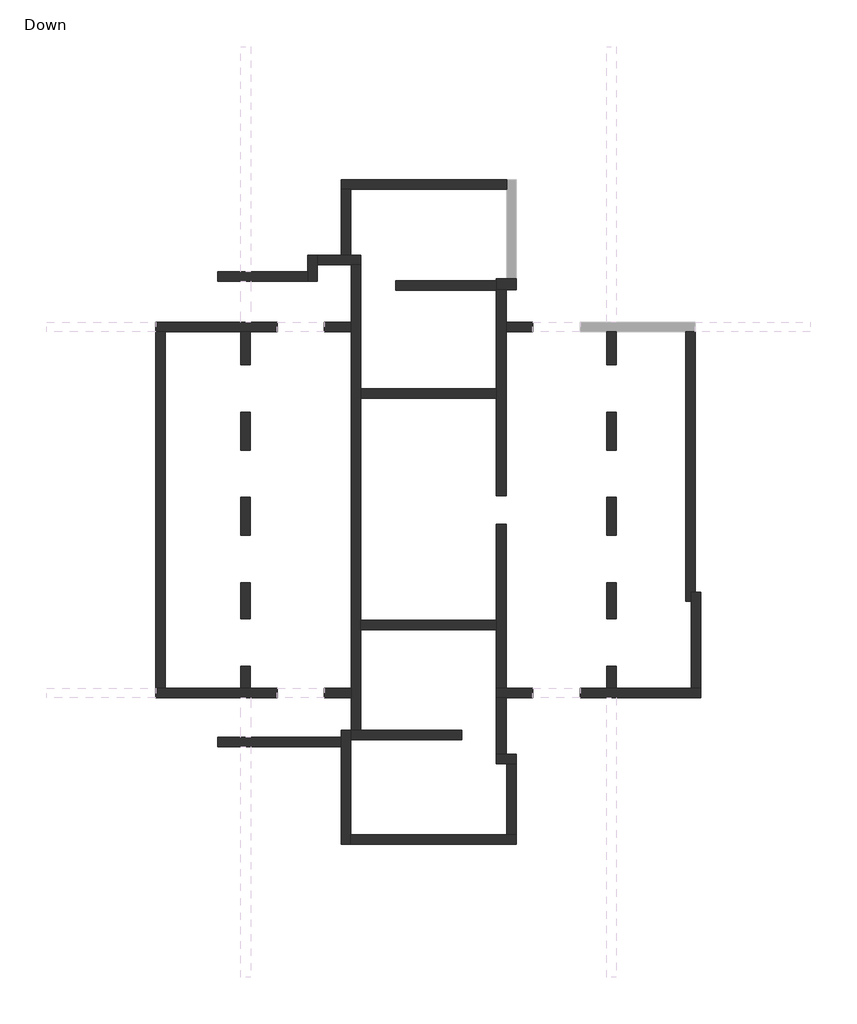
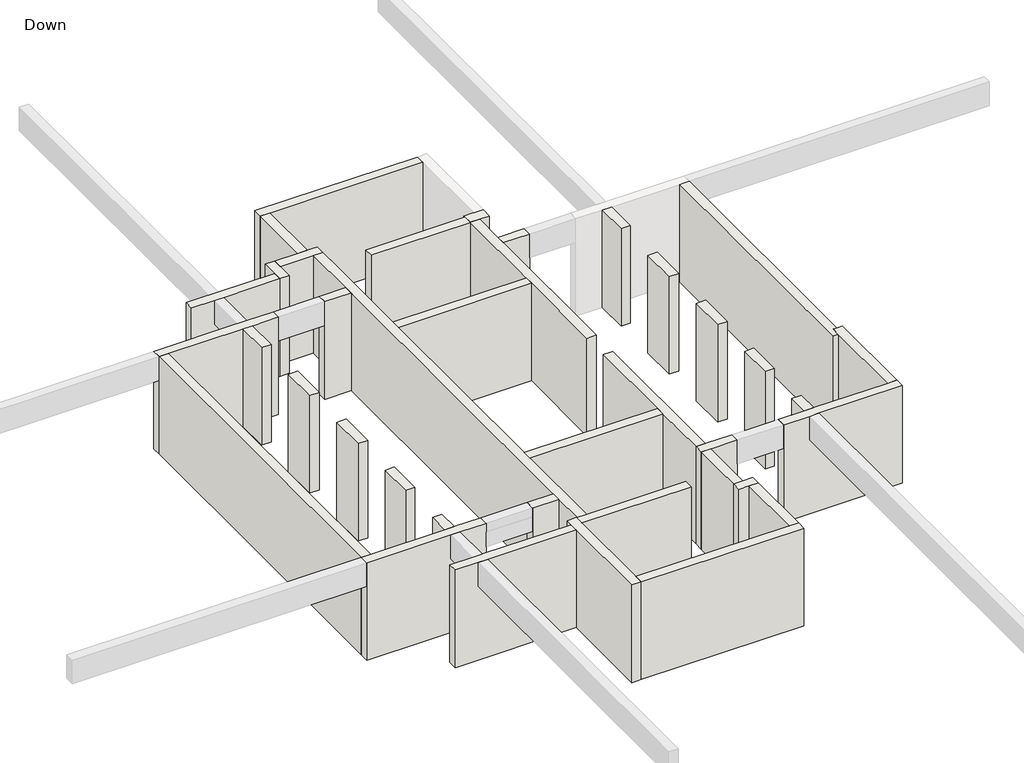
# One storey, part 1 of 2: 39 walls.
"""IFC4 building model written with IfcOpenShell, lengths in millimetres."""

from ifc_helpers import new_model, si_unit, origin, place, context, project, spatial, faceted_brep, element, save

model = new_model("IFC4")

# Units and contexts
model_context = context("Model", 3, world=origin())
ifc_project = project(units=[si_unit("LENGTHUNIT", "METRE", prefix="MILLI")], contexts=[model_context])

# Site, building, storey
site = spatial("IfcSite", under=ifc_project)
building = spatial("IfcBuilding", under=site)
storey = spatial("IfcBuildingStorey", under=building, Name="Down", Elevation=0.0)

# Walls
placement = place(None, origin())
element("IfcWall", 1, ObjectType="30", at=placement, inside=storey, context=model_context, shape_type="Brep", body=[
    faceted_brep([(-9097.9299438, -2256.2642878, 0.0), (-5277.5582989, -2256.2642878, 0.0), (-5277.5582989, -2256.2642878, 2500.0), (-5277.5582989, -2256.2642878, 3000.0), (-5277.5582989, -2256.2642878, 3300.0), (-6115.2243211, -2256.2642878, 3300.0), (-6415.2243211, -2256.2642878, 3300.0), (-9097.9299438, -2256.2642878, 3300.0), (-9097.9299438, -2256.2642878, 2500.0), (-9097.9299438, -1956.2642878, 0.0), (-9097.9299438, -1956.2642878, 2500.0), (-9097.9299438, -1956.2642878, 3300.0), (-8797.9299438, -1956.2642878, 3300.0), (-6419.4715818, -1956.2642878, 3300.0), (-6119.4715818, -1956.2642878, 3300.0), (-5277.5582989, -1956.2642878, 3300.0), (-5277.5582989, -1956.2642878, 2500.0), (-5277.5582989, -1956.2642878, 0.0), (-6119.4715818, -1956.2642878, 0.0), (-6419.4715818, -1956.2642878, 0.0), (-8797.9299438, -1956.2642878, 0.0), (-5277.5582989, -2251.2642878, 3300.0)], [[[0, 1, 2, 3, 4, 5, 6, 7, 8]], [[9, 10, 11, 12, 13, 14, 15, 16, 17, 18, 19, 20]], [[1, 0, 9, 20, 19, 18, 17]], [[4, 3, 2, 1, 17, 16, 15, 21]], [[7, 6, 5, 4, 21, 15, 14, 13, 12, 11]], [[0, 8, 7, 11, 10, 9]]]),
])
element("IfcWall", 2, ObjectType="30", at=placement, inside=storey, context=model_context, shape_type="Brep", body=[
    faceted_brep([(-3791.391747, -2256.2642878, 0.0), (-2947.5514166, -2256.2642878, 0.0), (-2947.5514166, -2256.2642878, 3000.0), (-2947.5514166, -2256.2642878, 3300.0), (-3791.391747, -2256.2642878, 3300.0), (-3791.391747, -2256.2642878, 3000.0), (-3791.391747, -2256.2642878, 2500.0), (-3791.391747, -1956.2642878, 0.0), (-3791.391747, -1956.2642878, 2500.0), (-3791.391747, -1956.2642878, 3300.0), (-2947.5514166, -1956.2642878, 3300.0), (-2947.5514166, -1956.2642878, 3000.0), (-2947.5514166, -1956.2642878, 0.0), (-3791.391747, -2251.2642878, 3300.0)], [[[0, 1, 2, 3, 4, 5, 6]], [[7, 8, 9, 10, 11, 12]], [[1, 0, 7, 12]], [[4, 3, 10, 9, 13]], [[0, 6, 5, 4, 13, 9, 8, 7]], [[3, 2, 1, 12, 11, 10]]]),
])
element("IfcWall", 3, ObjectType="30", at=placement, inside=storey, context=model_context, shape_type="Brep", body=[
    faceted_brep([(-2647.5514166, -3272.2312527, 0.0), (-2647.5514166, -123.5733036, 0.0), (-2647.5514166, 176.4266964, 0.0), (-2647.5514166, 7164.5202959, 0.0), (-2647.5514166, 7464.5202959, 0.0), (-2647.5514166, 11352.4074259, 0.0), (-2647.5514166, 11352.4074259, 3300.0), (-2647.5514166, 10558.9456228, 3300.0), (-2647.5514166, 7464.5202959, 3300.0), (-2647.5514166, 7164.5202959, 3300.0), (-2647.5514166, 176.4266964, 3300.0), (-2647.5514166, -123.5733036, 3300.0), (-2647.5514166, -3272.2312527, 3300.0), (-2947.5514166, -3272.2312527, 0.0), (-2947.5514166, -3272.2312527, 3000.0), (-2947.5514166, -3272.2312527, 3300.0), (-2947.5514166, -2256.2642878, 3300.0), (-2947.5514166, -1956.2642878, 3300.0), (-2947.5514166, 9251.0309634, 3300.0), (-2947.5514166, 9551.0309634, 3300.0), (-2947.5514166, 11352.4074259, 3300.0), (-2947.5514166, 11352.4074259, 3000.0), (-2947.5514166, 11352.4074259, 0.0), (-2947.5514166, 9551.0309634, 0.0), (-2947.5514166, 9251.0309634, 0.0), (-2947.5514166, -1956.2642878, 0.0), (-2947.5514166, -2256.2642878, 0.0)], [[[0, 1, 2, 3, 4, 5, 6, 7, 8, 9, 10, 11, 12]], [[13, 14, 15, 16, 17, 18, 19, 20, 21, 22, 23, 24, 25, 26]], [[5, 4, 3, 2, 1, 0, 13, 26, 25, 24, 23, 22]], [[12, 11, 10, 9, 8, 7, 6, 20, 19, 18, 17, 16, 15]], [[0, 12, 15, 14, 13]], [[6, 5, 22, 21, 20]]]),
])
element("IfcWall", 4, ObjectType="30", at=placement, inside=storey, context=model_context, shape_type="Brep", body=[
    faceted_brep([(-2947.5514166, 9551.0309634, 0.0), (-3791.391747, 9551.0309634, 0.0), (-3791.391747, 9551.0309634, 2500.0), (-3791.391747, 9551.0309634, 3300.0), (-2947.5514166, 9551.0309634, 3300.0), (-2947.5514166, 9551.0309634, 3000.0), (-2947.5514166, 9251.0309634, 0.0), (-2947.5514166, 9251.0309634, 3000.0), (-2947.5514166, 9251.0309634, 3300.0), (-3791.391747, 9251.0309634, 3300.0), (-3791.391747, 9251.0309634, 2500.0), (-3791.391747, 9251.0309634, 0.0)], [[[0, 1, 2, 3, 4, 5]], [[6, 7, 8, 9, 10, 11]], [[1, 0, 6, 11]], [[3, 2, 1, 11, 10, 9]], [[4, 3, 9, 8]], [[0, 5, 4, 8, 7, 6]]]),
])
element("IfcWall", 5, ObjectType="30", at=placement, inside=storey, context=model_context, shape_type="Brep", body=[
    faceted_brep([(-5277.5582989, 9551.0309634, 0.0), (-9097.9299438, 9551.0309634, 0.0), (-9097.9299438, 9551.0309634, 2500.0), (-9097.9299438, 9551.0309634, 3300.0), (-6415.2243211, 9551.0309634, 3300.0), (-6115.2243211, 9551.0309634, 3300.0), (-5277.5582989, 9551.0309634, 3300.0), (-5277.5582989, 9551.0309634, 2500.0), (-5277.5582989, 9251.0309634, 0.0), (-5277.5582989, 9251.0309634, 2500.0), (-5277.5582989, 9251.0309634, 3300.0), (-6119.4715818, 9251.0309634, 3300.0), (-6419.4715818, 9251.0309634, 3300.0), (-8797.9299438, 9251.0309634, 3300.0), (-9097.9299438, 9251.0309634, 3300.0), (-9097.9299438, 9251.0309634, 2500.0), (-9097.9299438, 9251.0309634, 0.0), (-8797.9299438, 9251.0309634, 0.0), (-6419.4715818, 9251.0309634, 0.0), (-6119.4715818, 9251.0309634, 0.0)], [[[0, 1, 2, 3, 4, 5, 6, 7]], [[8, 9, 10, 11, 12, 13, 14, 15, 16, 17, 18, 19]], [[1, 0, 8, 19, 18, 17, 16]], [[6, 5, 4, 3, 14, 13, 12, 11, 10]], [[0, 7, 6, 10, 9, 8]], [[3, 2, 1, 16, 15, 14]]]),
])
element("IfcWall", 6, ObjectType="30", at=placement, inside=storey, context=model_context, shape_type="Brep", body=[
    faceted_brep([(-9097.9299438, 9251.0309634, 0.0), (-9097.9299438, -1956.2642878, 0.0), (-9097.9299438, -1956.2642878, 3000.0), (-9097.9299438, -1956.2642878, 3300.0), (-9097.9299438, 9251.0309634, 3300.0), (-9097.9299438, 9251.0309634, 3000.0), (-8797.9299438, 9251.0309634, 0.0), (-8797.9299438, 9251.0309634, 3300.0), (-8797.9299438, -1956.2642878, 3300.0), (-8797.9299438, -1956.2642878, 0.0)], [[[0, 1, 2, 3, 4, 5]], [[6, 7, 8, 9]], [[1, 0, 6, 9]], [[4, 3, 8, 7]], [[3, 2, 1, 9, 8]], [[0, 5, 4, 7, 6]]]),
])
element("IfcWall", 7, ObjectType="30", at=placement, inside=storey, context=model_context, shape_type="Brep", body=[
    faceted_brep([(-6119.4715818, -1956.2642878, 0.0), (-6119.4715818, -1265.4865865, 0.0), (-6119.4715818, -1265.4865865, 3000.0), (-6119.4715818, -1265.4865865, 3300.0), (-6119.4715818, -1956.2642878, 3300.0), (-6119.4715818, -1956.2642878, 3000.0), (-6419.4715818, -1956.2642878, 0.0), (-6419.4715818, -1956.2642878, 3300.0), (-6419.4715818, -1265.4865865, 3300.0), (-6419.4715818, -1265.4865865, 3000.0), (-6419.4715818, -1265.4865865, 0.0)], [[[0, 1, 2, 3, 4, 5]], [[6, 7, 8, 9, 10]], [[1, 0, 6, 10]], [[3, 2, 1, 10, 9, 8]], [[4, 3, 8, 7]], [[0, 5, 4, 7, 6]]]),
])
element("IfcWall", 8, ObjectType="30", at=placement, inside=storey, context=model_context, shape_type="Brep", body=[
    faceted_brep([(-6119.4715818, 224.8781761, 0.0), (-6119.4715818, 1362.5932484, 0.0), (-6119.4715818, 1362.5932484, 3000.0), (-6119.4715818, 1362.5932484, 3300.0), (-6119.4715818, 224.8781761, 3300.0), (-6119.4715818, 224.8781761, 3000.0), (-6419.4715818, 224.8781761, 0.0), (-6419.4715818, 224.8781761, 3000.0), (-6419.4715818, 224.8781761, 3300.0), (-6419.4715818, 1362.5932484, 3300.0), (-6419.4715818, 1362.5932484, 3000.0), (-6419.4715818, 1362.5932484, 0.0)], [[[0, 1, 2, 3, 4, 5]], [[6, 7, 8, 9, 10, 11]], [[1, 0, 6, 11]], [[3, 2, 1, 11, 10, 9]], [[4, 3, 9, 8]], [[0, 5, 4, 8, 7, 6]]]),
])
element("IfcWall", 9, ObjectType="30", at=placement, inside=storey, context=model_context, shape_type="Brep", body=[
    faceted_brep([(-6119.4715818, 2852.9580109, 0.0), (-6119.4715818, 4041.0516104, 0.0), (-6119.4715818, 4041.0516104, 3000.0), (-6119.4715818, 4041.0516104, 3300.0), (-6119.4715818, 2852.9580109, 3300.0), (-6119.4715818, 2852.9580109, 3000.0), (-6419.4715818, 2852.9580109, 0.0), (-6419.4715818, 2852.9580109, 3000.0), (-6419.4715818, 2852.9580109, 3300.0), (-6419.4715818, 4041.0516104, 3300.0), (-6419.4715818, 4041.0516104, 3000.0), (-6419.4715818, 4041.0516104, 0.0)], [[[0, 1, 2, 3, 4, 5]], [[6, 7, 8, 9, 10, 11]], [[1, 0, 6, 11]], [[3, 2, 1, 11, 10, 9]], [[4, 3, 9, 8]], [[0, 5, 4, 8, 7, 6]]]),
])
element("IfcWall", 10, ObjectType="30", at=placement, inside=storey, context=model_context, shape_type="Brep", body=[
    faceted_brep([(-6119.4715818, 5531.4163729, 0.0), (-6119.4715818, 6719.5099724, 0.0), (-6119.4715818, 6719.5099724, 3000.0), (-6119.4715818, 6719.5099724, 3300.0), (-6119.4715818, 5531.4163729, 3300.0), (-6119.4715818, 5531.4163729, 3000.0), (-6419.4715818, 5531.4163729, 0.0), (-6419.4715818, 5531.4163729, 3000.0), (-6419.4715818, 5531.4163729, 3300.0), (-6419.4715818, 6719.5099724, 3300.0), (-6419.4715818, 6719.5099724, 3000.0), (-6419.4715818, 6719.5099724, 0.0)], [[[0, 1, 2, 3, 4, 5]], [[6, 7, 8, 9, 10, 11]], [[1, 0, 6, 11]], [[3, 2, 1, 11, 10, 9]], [[4, 3, 9, 8]], [[0, 5, 4, 8, 7, 6]]]),
])
element("IfcWall", 11, ObjectType="30", at=placement, inside=storey, context=model_context, shape_type="Brep", body=[
    faceted_brep([(-6119.4715818, 8205.6765243, 0.0), (-6119.4715818, 9251.0309634, 0.0), (-6119.4715818, 9251.0309634, 3000.0), (-6119.4715818, 9251.0309634, 3300.0), (-6119.4715818, 8205.6765243, 3300.0), (-6119.4715818, 8205.6765243, 3000.0), (-6419.4715818, 8205.6765243, 0.0), (-6419.4715818, 8205.6765243, 3000.0), (-6419.4715818, 8205.6765243, 3300.0), (-6419.4715818, 9251.0309634, 3300.0), (-6419.4715818, 9251.0309634, 0.0)], [[[0, 1, 2, 3, 4, 5]], [[6, 7, 8, 9, 10]], [[1, 0, 6, 10]], [[4, 3, 9, 8]], [[0, 5, 4, 8, 7, 6]], [[3, 2, 1, 10, 9]]]),
])
element("IfcWall", 12, ObjectType="30", at=placement, inside=storey, context=model_context, shape_type="Brep", body=[
    faceted_brep([(8042.8271106, -1956.2642878, 0.0), (7742.8271106, -1956.2642878, 0.0), (5384.3687486, -1956.2642878, 0.0), (5084.3687486, -1956.2642878, 0.0), (4242.4554657, -1956.2642878, 0.0), (4242.4554657, -1956.2642878, 2500.0), (4242.4554657, -1956.2642878, 3300.0), (5084.3687486, -1956.2642878, 3300.0), (5384.3687486, -1956.2642878, 3300.0), (7742.8271106, -1956.2642878, 3300.0), (8042.8271106, -1956.2642878, 3300.0), (8042.8271106, -1956.2642878, 2500.0), (8042.8271106, -2256.2642878, 0.0), (8042.8271106, -2256.2642878, 2500.0), (8042.8271106, -2256.2642878, 3300.0), (5373.25294, -2256.2642878, 3300.0), (5073.25294, -2256.2642878, 3300.0), (4242.4554657, -2256.2642878, 3300.0), (4242.4554657, -2256.2642878, 2500.0), (4242.4554657, -2256.2642878, 0.0)], [[[0, 1, 2, 3, 4, 5, 6, 7, 8, 9, 10, 11]], [[12, 13, 14, 15, 16, 17, 18, 19]], [[4, 3, 2, 1, 0, 12, 19]], [[6, 5, 4, 19, 18, 17]], [[10, 9, 8, 7, 6, 17, 16, 15, 14]], [[0, 11, 10, 14, 13, 12]]]),
])
element("IfcWall", 13, ObjectType="30", at=placement, inside=storey, context=model_context, shape_type="Brep", body=[
    faceted_brep([(2756.2889137, -1956.2642878, 0.0), (1915.9035042, -1956.2642878, 0.0), (1615.9035042, -1956.2642878, 0.0), (1615.9035042, -1956.2642878, 3300.0), (1915.9035042, -1956.2642878, 3300.0), (2756.2889137, -1956.2642878, 3300.0), (2756.2889137, -1956.2642878, 2500.0), (2756.2889137, -2256.2642878, 0.0), (2756.2889137, -2256.2642878, 2500.0), (2756.2889137, -2256.2642878, 3300.0), (1915.9035042, -2256.2642878, 3300.0), (1615.9035042, -2256.2642878, 3300.0), (1615.9035042, -2256.2642878, 0.0), (1915.9035042, -2256.2642878, 0.0)], [[[0, 1, 2, 3, 4, 5, 6]], [[7, 8, 9, 10, 11, 12, 13]], [[2, 1, 0, 7, 13, 12]], [[5, 4, 3, 11, 10, 9]], [[0, 6, 5, 9, 8, 7]], [[3, 2, 12, 11]]]),
])
element("IfcWall", 14, ObjectType="30", at=placement, inside=storey, context=model_context, shape_type="Brep", body=[
    faceted_brep([(1915.9035042, -1956.2642878, 0.0), (1915.9035042, 3193.7357122, 0.0), (1915.9035042, 3193.7357122, 3000.0), (1915.9035042, 3193.7357122, 3300.0), (1915.9035042, -1956.2642878, 3300.0), (1915.9035042, -1956.2642878, 3000.0), (1615.9035042, -1956.2642878, 0.0), (1615.9035042, -1956.2642878, 3300.0), (1615.9035042, -123.5733036, 3300.0), (1615.9035042, 176.4266964, 3300.0), (1615.9035042, 3193.7357122, 3300.0), (1615.9035042, 3193.7357122, 3000.0), (1615.9035042, 3193.7357122, 0.0), (1615.9035042, 176.4266964, 0.0), (1615.9035042, -123.5733036, 0.0)], [[[0, 1, 2, 3, 4, 5]], [[6, 7, 8, 9, 10, 11, 12, 13, 14]], [[1, 0, 6, 14, 13, 12]], [[3, 2, 1, 12, 11, 10]], [[4, 3, 10, 9, 8, 7]], [[0, 5, 4, 7, 6]]]),
])
element("IfcWall", 15, ObjectType="30", at=placement, inside=storey, context=model_context, shape_type="Brep", body=[
    faceted_brep([(1915.9035042, 9251.0309634, 0.0), (2756.2889137, 9251.0309634, 0.0), (2756.2889137, 9251.0309634, 2500.0), (2756.2889137, 9251.0309634, 3300.0), (1915.9035042, 9251.0309634, 3300.0), (1915.9035042, 9251.0309634, 3000.0), (1915.9035042, 9551.0309634, 0.0), (1915.9035042, 9551.0309634, 3000.0), (1915.9035042, 9551.0309634, 3300.0), (2756.2889137, 9551.0309634, 3300.0), (2756.2889137, 9551.0309634, 2500.0), (2756.2889137, 9551.0309634, 0.0)], [[[0, 1, 2, 3, 4, 5]], [[6, 7, 8, 9, 10, 11]], [[1, 0, 6, 11]], [[3, 2, 1, 11, 10, 9]], [[4, 3, 9, 8]], [[0, 5, 4, 8, 7, 6]]]),
])
element("IfcWall", 16, ObjectType="30", at=placement, inside=storey, context=model_context, shape_type="Brep", body=[
    faceted_brep([(7742.8271106, 1064.5202959, 0.0), (7742.8271106, 771.0309634, 0.0), (7742.8271106, -1956.2642878, 0.0), (7742.8271106, -1956.2642878, 3300.0), (7742.8271106, 771.0309634, 3300.0), (7742.8271106, 1064.5202959, 3300.0), (8042.8271106, 1064.5202959, 0.0), (8042.8271106, 1064.5202959, 3000.0), (8042.8271106, 1064.5202959, 3300.0), (8042.8271106, -1956.2642878, 3300.0), (8042.8271106, -1956.2642878, 3000.0), (8042.8271106, -1956.2642878, 0.0), (7862.8408752, 1064.5202959, 0.0), (7862.8408752, 1064.5202959, 3300.0)], [[[0, 1, 2, 3, 4, 5]], [[6, 7, 8, 9, 10, 11]], [[2, 1, 0, 12, 6, 11]], [[5, 4, 3, 9, 8, 13]], [[0, 5, 13, 8, 7, 6, 12]], [[3, 2, 11, 10, 9]]]),
])
element("IfcWall", 17, ObjectType="30", at=placement, inside=storey, context=model_context, shape_type="Brep", body=[
    faceted_brep([(5384.3687486, -1956.2642878, 0.0), (5384.3687486, -1265.4865865, 0.0), (5384.3687486, -1265.4865865, 3000.0), (5384.3687486, -1265.4865865, 3300.0), (5384.3687486, -1956.2642878, 3300.0), (5084.3687486, -1956.2642878, 0.0), (5084.3687486, -1956.2642878, 3000.0), (5084.3687486, -1956.2642878, 3300.0), (5084.3687486, -1265.4865865, 3300.0), (5084.3687486, -1265.4865865, 3000.0), (5084.3687486, -1265.4865865, 0.0)], [[[0, 1, 2, 3, 4]], [[5, 6, 7, 8, 9, 10]], [[1, 0, 5, 10]], [[3, 2, 1, 10, 9, 8]], [[4, 3, 8, 7]], [[0, 4, 7, 6, 5]]]),
])
element("IfcWall", 18, ObjectType="30", at=placement, inside=storey, context=model_context, shape_type="Brep", body=[
    faceted_brep([(5384.3687486, 224.8781761, 0.0), (5384.3687486, 1362.5932484, 0.0), (5384.3687486, 1362.5932484, 3000.0), (5384.3687486, 1362.5932484, 3300.0), (5384.3687486, 224.8781761, 3300.0), (5384.3687486, 224.8781761, 3000.0), (5084.3687486, 224.8781761, 0.0), (5084.3687486, 224.8781761, 3000.0), (5084.3687486, 224.8781761, 3300.0), (5084.3687486, 1362.5932484, 3300.0), (5084.3687486, 1362.5932484, 3000.0), (5084.3687486, 1362.5932484, 0.0)], [[[0, 1, 2, 3, 4, 5]], [[6, 7, 8, 9, 10, 11]], [[1, 0, 6, 11]], [[3, 2, 1, 11, 10, 9]], [[4, 3, 9, 8]], [[0, 5, 4, 8, 7, 6]]]),
])
element("IfcWall", 19, ObjectType="30", at=placement, inside=storey, context=model_context, shape_type="Brep", body=[
    faceted_brep([(5384.3687486, 2852.9580109, 0.0), (5384.3687486, 4041.0516104, 0.0), (5384.3687486, 4041.0516104, 3000.0), (5384.3687486, 4041.0516104, 3300.0), (5384.3687486, 2852.9580109, 3300.0), (5384.3687486, 2852.9580109, 3000.0), (5084.3687486, 2852.9580109, 0.0), (5084.3687486, 2852.9580109, 3000.0), (5084.3687486, 2852.9580109, 3300.0), (5084.3687486, 4041.0516104, 3300.0), (5084.3687486, 4041.0516104, 3000.0), (5084.3687486, 4041.0516104, 0.0)], [[[0, 1, 2, 3, 4, 5]], [[6, 7, 8, 9, 10, 11]], [[1, 0, 6, 11]], [[3, 2, 1, 11, 10, 9]], [[4, 3, 9, 8]], [[0, 5, 4, 8, 7, 6]]]),
])
element("IfcWall", 20, ObjectType="30", at=placement, inside=storey, context=model_context, shape_type="Brep", body=[
    faceted_brep([(5384.3687486, 5531.4163729, 0.0), (5384.3687486, 6719.5099724, 0.0), (5384.3687486, 6719.5099724, 3000.0), (5384.3687486, 6719.5099724, 3300.0), (5384.3687486, 5531.4163729, 3300.0), (5384.3687486, 5531.4163729, 3000.0), (5084.3687486, 5531.4163729, 0.0), (5084.3687486, 5531.4163729, 3000.0), (5084.3687486, 5531.4163729, 3300.0), (5084.3687486, 6719.5099724, 3300.0), (5084.3687486, 6719.5099724, 3000.0), (5084.3687486, 6719.5099724, 0.0)], [[[0, 1, 2, 3, 4, 5]], [[6, 7, 8, 9, 10, 11]], [[1, 0, 6, 11]], [[3, 2, 1, 11, 10, 9]], [[4, 3, 9, 8]], [[0, 5, 4, 8, 7, 6]]]),
])
element("IfcWall", 21, ObjectType="30", at=placement, inside=storey, context=model_context, shape_type="Brep", body=[
    faceted_brep([(5384.3687486, 8205.6765243, 0.0), (5384.3687486, 9251.0309634, 0.0), (5384.3687486, 9251.0309634, 3300.0), (5384.3687486, 8205.6765243, 3300.0), (5384.3687486, 8205.6765243, 3000.0), (5084.3687486, 8205.6765243, 0.0), (5084.3687486, 8205.6765243, 3000.0), (5084.3687486, 8205.6765243, 3300.0), (5084.3687486, 9251.0309634, 3300.0), (5084.3687486, 9251.0309634, 3000.0), (5084.3687486, 9251.0309634, 0.0)], [[[0, 1, 2, 3, 4]], [[5, 6, 7, 8, 9, 10]], [[1, 0, 5, 10]], [[3, 2, 8, 7]], [[0, 4, 3, 7, 6, 5]], [[2, 1, 10, 9, 8]]]),
])
element("IfcWall", 22, ObjectType="30", at=placement, inside=storey, context=model_context, shape_type="Brep", body=[
    faceted_brep([(7562.8408752, 9251.0309634, 0.0), (7562.8408752, 771.0309634, 0.0), (7562.8408752, 771.0309634, 3300.0), (7562.8408752, 9251.0309634, 3300.0), (7862.8408752, 9251.0309634, 0.0), (7862.8408752, 9251.0309634, 3000.0), (7862.8408752, 9251.0309634, 3300.0), (7862.8408752, 1064.5202959, 3300.0), (7862.8408752, 1064.5202959, 3000.0), (7862.8408752, 1064.5202959, 0.0), (7742.8271106, 1064.5202959, 0.0), (7742.8271106, 771.0309634, 0.0), (7742.8271106, 771.0309634, 3300.0), (7742.8271106, 1064.5202959, 3300.0)], [[[0, 1, 2, 3]], [[4, 5, 6, 7, 8, 9]], [[1, 0, 4, 9, 10, 11]], [[2, 1, 11, 12]], [[3, 2, 12, 13, 7, 6]], [[0, 3, 6, 5, 4]], [[10, 13, 12, 11]], [[13, 10, 9, 8, 7]]]),
])
element("IfcWall", 23, ObjectType="30", at=placement, inside=storey, context=model_context, shape_type="Brep", body=[
    faceted_brep([(-2647.5514166, -123.5733036, 0.0), (1615.9035042, -123.5733036, 0.0), (1615.9035042, -123.5733036, 3300.0), (-2647.5514166, -123.5733036, 3300.0), (-2647.5514166, 176.4266964, 0.0), (-2647.5514166, 176.4266964, 3000.0), (-2647.5514166, 176.4266964, 3300.0), (1615.9035042, 176.4266964, 3300.0), (1615.9035042, 176.4266964, 3000.0), (1615.9035042, 176.4266964, 0.0)], [[[0, 1, 2, 3]], [[4, 5, 6, 7, 8, 9]], [[1, 0, 4, 9]], [[3, 2, 7, 6]], [[0, 3, 6, 5, 4]], [[2, 1, 9, 8, 7]]]),
])
element("IfcWall", 24, ObjectType="30", at=placement, inside=storey, context=model_context, shape_type="Brep", body=[
    faceted_brep([(-7145.7620154, -3792.8093669, 0.0), (-3270.8136327, -3792.8093669, 0.0), (-3270.8136327, -3792.8093669, 3000.0), (-3270.8136327, -3792.8093669, 3300.0), (-6115.2243211, -3792.8093669, 3300.0), (-6415.2243211, -3792.8093669, 3300.0), (-7145.7620154, -3792.8093669, 3300.0), (-7145.7620154, -3792.8093669, 3000.0), (-7145.7620154, -3492.8093669, 0.0), (-7145.7620154, -3492.8093669, 3000.0), (-7145.7620154, -3492.8093669, 3300.0), (-6415.2243211, -3492.8093669, 3300.0), (-6115.2243211, -3492.8093669, 3300.0), (-3270.8136327, -3492.8093669, 3300.0), (-3270.8136327, -3492.8093669, 3000.0), (-3270.8136327, -3492.8093669, 0.0)], [[[0, 1, 2, 3, 4, 5, 6, 7]], [[8, 9, 10, 11, 12, 13, 14, 15]], [[1, 0, 8, 15]], [[6, 5, 4, 3, 13, 12, 11, 10]], [[0, 7, 6, 10, 9, 8]], [[3, 2, 1, 15, 14, 13]]]),
])
element("IfcWall", 25, ObjectType="30", at=placement, inside=storey, context=model_context, shape_type="Brep", body=[
    faceted_brep([(-3270.8136327, -3272.2312527, 0.0), (-3270.8136327, -3492.8093669, 0.0), (-3270.8136327, -3792.8093669, 0.0), (-3270.8136327, -6865.8995252, 0.0), (-3270.8136327, -6865.8995252, 3000.0), (-3270.8136327, -6865.8995252, 3300.0), (-3270.8136327, -3792.8093669, 3300.0), (-3270.8136327, -3492.8093669, 3300.0), (-3270.8136327, -3272.2312527, 3300.0), (-3270.8136327, -3272.2312527, 3000.0), (-2970.8136327, -3272.2312527, 0.0), (-2970.8136327, -3272.2312527, 3300.0), (-2970.8136327, -3572.2312527, 3300.0), (-2970.8136327, -6565.8995252, 3300.0), (-2970.8136327, -6865.8995252, 3300.0), (-2970.8136327, -6865.8995252, 0.0), (-2970.8136327, -6565.8995252, 0.0), (-2970.8136327, -3572.2312527, 0.0)], [[[0, 1, 2, 3, 4, 5, 6, 7, 8, 9]], [[10, 11, 12, 13, 14, 15, 16, 17]], [[3, 2, 1, 0, 10, 17, 16, 15]], [[8, 7, 6, 5, 14, 13, 12, 11]], [[5, 4, 3, 15, 14]], [[0, 9, 8, 11, 10]]]),
])
element("IfcWall", 26, ObjectType="30", at=placement, inside=storey, context=model_context, shape_type="Brep", body=[
    faceted_brep([(-2970.8136327, -6865.8995252, 0.0), (2233.0404623, -6865.8995252, 0.0), (2233.0404623, -6865.8995252, 3000.0), (2233.0404623, -6865.8995252, 3300.0), (-2970.8136327, -6865.8995252, 3300.0), (-2970.8136327, -6565.8995252, 0.0), (-2970.8136327, -6565.8995252, 3000.0), (-2970.8136327, -6565.8995252, 3300.0), (1933.0404623, -6565.8995252, 3300.0), (2233.0404623, -6565.8995252, 3300.0), (2233.0404623, -6565.8995252, 0.0), (1933.0404623, -6565.8995252, 0.0)], [[[0, 1, 2, 3, 4]], [[5, 6, 7, 8, 9, 10, 11]], [[1, 0, 5, 11, 10]], [[4, 3, 9, 8, 7]], [[0, 4, 7, 6, 5]], [[3, 2, 1, 10, 9]]]),
])
element("IfcWall", 27, ObjectType="30", at=placement, inside=storey, context=model_context, shape_type="Brep", body=[
    faceted_brep([(2233.0404623, -6565.8995252, 0.0), (2233.0404623, -4336.2642878, 0.0), (2233.0404623, -4336.2642878, 3300.0), (2233.0404623, -6565.8995252, 3300.0), (1933.0404623, -6565.8995252, 0.0), (1933.0404623, -6565.8995252, 3000.0), (1933.0404623, -6565.8995252, 3300.0), (1933.0404623, -4336.2642878, 3300.0), (1933.0404623, -4336.2642878, 3000.0), (1933.0404623, -4336.2642878, 0.0)], [[[0, 1, 2, 3]], [[4, 5, 6, 7, 8, 9]], [[1, 0, 4, 9]], [[3, 2, 7, 6]], [[0, 3, 6, 5, 4]], [[2, 1, 9, 8, 7]]]),
])
element("IfcWall", 28, ObjectType="30", at=placement, inside=storey, context=model_context, shape_type="Brep", body=[
    faceted_brep([(1615.9035042, -2256.2642878, 0.0), (1615.9035042, -4036.2642878, 0.0), (1615.9035042, -4036.2642878, 3300.0), (1615.9035042, -3272.2312527, 3300.0), (1615.9035042, -2256.2642878, 3300.0), (1915.9035042, -2256.2642878, 0.0), (1915.9035042, -2256.2642878, 3000.0), (1915.9035042, -2256.2642878, 3300.0), (1915.9035042, -4036.2642878, 3300.0), (1915.9035042, -4036.2642878, 3000.0), (1915.9035042, -4036.2642878, 0.0)], [[[0, 1, 2, 3, 4]], [[5, 6, 7, 8, 9, 10]], [[1, 0, 5, 10]], [[4, 3, 2, 8, 7]], [[0, 4, 7, 6, 5]], [[2, 1, 10, 9, 8]]]),
])
element("IfcWall", 29, ObjectType="30", at=placement, inside=storey, context=model_context, shape_type="Brep", body=[
    faceted_brep([(1615.9035042, -4336.2642878, 0.0), (1933.0404623, -4336.2642878, 0.0), (2233.0404623, -4336.2642878, 0.0), (2233.0404623, -4336.2642878, 3300.0), (1933.0404623, -4336.2642878, 3300.0), (1615.9035042, -4336.2642878, 3300.0), (1615.9035042, -4336.2642878, 3000.0), (1615.9035042, -4036.2642878, 0.0), (1615.9035042, -4036.2642878, 3300.0), (1915.9035042, -4036.2642878, 3300.0), (2233.0404623, -4036.2642878, 3300.0), (2233.0404623, -4036.2642878, 3000.0), (2233.0404623, -4036.2642878, 0.0), (1915.9035042, -4036.2642878, 0.0)], [[[0, 1, 2, 3, 4, 5, 6]], [[7, 8, 9, 10, 11, 12, 13]], [[2, 1, 0, 7, 13, 12]], [[5, 4, 3, 10, 9, 8]], [[0, 6, 5, 8, 7]], [[3, 2, 12, 11, 10]]]),
])
element("IfcWall", 30, ObjectType="30", at=placement, inside=storey, context=model_context, shape_type="Brep", body=[
    faceted_brep([(1915.9035042, 4091.4301376, 0.0), (1915.9035042, 9251.0309634, 0.0), (1915.9035042, 9551.0309634, 0.0), (1915.9035042, 10565.0708809, 0.0), (1915.9035042, 10565.0708809, 3000.0), (1915.9035042, 10565.0708809, 3300.0), (1915.9035042, 9551.0309634, 3300.0), (1915.9035042, 9251.0309634, 3300.0), (1915.9035042, 4091.4301376, 3300.0), (1915.9035042, 4091.4301376, 3000.0), (1615.9035042, 4091.4301376, 0.0), (1615.9035042, 4091.4301376, 3000.0), (1615.9035042, 4091.4301376, 3300.0), (1615.9035042, 7164.5202959, 3300.0), (1615.9035042, 7464.5202959, 3300.0), (1615.9035042, 10558.9456228, 3300.0), (1615.9035042, 10565.0708809, 3300.0), (1615.9035042, 10565.0708809, 0.0), (1615.9035042, 10558.9456228, 0.0), (1615.9035042, 7464.5202959, 0.0), (1615.9035042, 7164.5202959, 0.0)], [[[0, 1, 2, 3, 4, 5, 6, 7, 8, 9]], [[10, 11, 12, 13, 14, 15, 16, 17, 18, 19, 20]], [[3, 2, 1, 0, 10, 20, 19, 18, 17]], [[8, 7, 6, 5, 16, 15, 14, 13, 12]], [[0, 9, 8, 12, 11, 10]], [[5, 4, 3, 17, 16]]]),
])
element("IfcWall", 31, ObjectType="30", at=placement, inside=storey, context=model_context, shape_type="Brep", body=[
    faceted_brep([(-2647.5514166, 7164.5202959, 0.0), (1615.9035042, 7164.5202959, 0.0), (1615.9035042, 7164.5202959, 3000.0), (1615.9035042, 7164.5202959, 3300.0), (-2647.5514166, 7164.5202959, 3300.0), (-2647.5514166, 7164.5202959, 3000.0), (-2647.5514166, 7464.5202959, 0.0), (-2647.5514166, 7464.5202959, 3300.0), (1615.9035042, 7464.5202959, 3300.0), (1615.9035042, 7464.5202959, 0.0)], [[[0, 1, 2, 3, 4, 5]], [[6, 7, 8, 9]], [[1, 0, 6, 9]], [[4, 3, 8, 7]], [[0, 5, 4, 7, 6]], [[3, 2, 1, 9, 8]]]),
])
element("IfcWall", 32, ObjectType="30", at=placement, inside=storey, context=model_context, shape_type="Brep", body=[
    faceted_brep([(1933.0404623, 14032.7928354, 0.0), (-3270.8136327, 14032.7928354, 0.0), (-3270.8136327, 14032.7928354, 3000.0), (-3270.8136327, 14032.7928354, 3300.0), (1933.0404623, 14032.7928354, 3300.0), (1933.0404623, 13732.7928354, 0.0), (1933.0404623, 13732.7928354, 3000.0), (1933.0404623, 13732.7928354, 3300.0), (-2970.8136327, 13732.7928354, 3300.0), (-3270.8136327, 13732.7928354, 3300.0), (-3270.8136327, 13732.7928354, 0.0), (-2970.8136327, 13732.7928354, 0.0)], [[[0, 1, 2, 3, 4]], [[5, 6, 7, 8, 9, 10, 11]], [[1, 0, 5, 11, 10]], [[4, 3, 9, 8, 7]], [[0, 4, 7, 6, 5]], [[3, 2, 1, 10, 9]]]),
])
element("IfcWall", 33, ObjectType="30", at=placement, inside=storey, context=model_context, shape_type="Brep", body=[
    faceted_brep([(-3270.8136327, 13732.7928354, 0.0), (-3270.8136327, 11652.4074259, 0.0), (-3270.8136327, 11652.4074259, 3000.0), (-3270.8136327, 11652.4074259, 3300.0), (-3270.8136327, 13732.7928354, 3300.0), (-2970.8136327, 13732.7928354, 0.0), (-2970.8136327, 13732.7928354, 3000.0), (-2970.8136327, 13732.7928354, 3300.0), (-2970.8136327, 11652.4074259, 3300.0), (-2970.8136327, 11652.4074259, 3000.0), (-2970.8136327, 11652.4074259, 0.0)], [[[0, 1, 2, 3, 4]], [[5, 6, 7, 8, 9, 10]], [[1, 0, 5, 10]], [[4, 3, 8, 7]], [[0, 4, 7, 6, 5]], [[3, 2, 1, 10, 9, 8]]]),
])
element("IfcWall", 34, ObjectType="30", at=placement, inside=storey, context=model_context, shape_type="Brep", body=[
    faceted_brep([(-2647.5514166, 11652.4074259, 0.0), (-2970.8136327, 11652.4074259, 0.0), (-3270.8136327, 11652.4074259, 0.0), (-4013.8969087, 11652.4074259, 0.0), (-4013.8969087, 11652.4074259, 3300.0), (-3270.8136327, 11652.4074259, 3300.0), (-2970.8136327, 11652.4074259, 3300.0), (-2647.5514166, 11652.4074259, 3300.0), (-2647.5514166, 11652.4074259, 3000.0), (-2647.5514166, 11352.4074259, 0.0), (-2647.5514166, 11352.4074259, 3300.0), (-2947.5514166, 11352.4074259, 3300.0), (-4013.8969087, 11352.4074259, 3300.0), (-4013.8969087, 11352.4074259, 3000.0), (-4013.8969087, 11352.4074259, 0.0), (-2947.5514166, 11352.4074259, 0.0)], [[[0, 1, 2, 3, 4, 5, 6, 7, 8]], [[9, 10, 11, 12, 13, 14, 15]], [[3, 2, 1, 0, 9, 15, 14]], [[7, 6, 5, 4, 12, 11, 10]], [[4, 3, 14, 13, 12]], [[0, 8, 7, 10, 9]]]),
])
element("IfcWall", 35, ObjectType="30", at=placement, inside=storey, context=model_context, shape_type="Brep", body=[
    faceted_brep([(-4013.8969087, 10837.9545698, 0.0), (-4013.8969087, 11352.4074259, 0.0), (-4013.8969087, 11652.4074259, 0.0), (-4013.8969087, 11652.4074259, 3300.0), (-4013.8969087, 11352.4074259, 3300.0), (-4013.8969087, 10837.9545698, 3300.0), (-4013.8969087, 10837.9545698, 3000.0), (-4313.8969087, 10837.9545698, 0.0), (-4313.8969087, 10837.9545698, 3300.0), (-4313.8969087, 11137.9545698, 3300.0), (-4313.8969087, 11652.4074259, 3300.0), (-4313.8969087, 11652.4074259, 3000.0), (-4313.8969087, 11652.4074259, 0.0), (-4313.8969087, 11137.9545698, 0.0)], [[[0, 1, 2, 3, 4, 5, 6]], [[7, 8, 9, 10, 11, 12, 13]], [[2, 1, 0, 7, 13, 12]], [[5, 4, 3, 10, 9, 8]], [[3, 2, 12, 11, 10]], [[0, 6, 5, 8, 7]]]),
])
element("IfcWall", 36, ObjectType="30", at=placement, inside=storey, context=model_context, shape_type="Brep", body=[
    faceted_brep([(-4313.8969087, 11137.9545698, 0.0), (-7145.7620154, 11137.9545698, 0.0), (-7145.7620154, 11137.9545698, 3000.0), (-7145.7620154, 11137.9545698, 3300.0), (-6415.2243211, 11137.9545698, 3300.0), (-6115.2243211, 11137.9545698, 3300.0), (-4313.8969087, 11137.9545698, 3300.0), (-4313.8969087, 11137.9545698, 3000.0), (-4313.8969087, 10837.9545698, 0.0), (-4313.8969087, 10837.9545698, 3300.0), (-6115.2243211, 10837.9545698, 3300.0), (-6415.2243211, 10837.9545698, 3300.0), (-7145.7620154, 10837.9545698, 3300.0), (-7145.7620154, 10837.9545698, 3000.0), (-7145.7620154, 10837.9545698, 0.0)], [[[0, 1, 2, 3, 4, 5, 6, 7]], [[8, 9, 10, 11, 12, 13, 14]], [[1, 0, 8, 14]], [[3, 2, 1, 14, 13, 12]], [[6, 5, 4, 3, 12, 11, 10, 9]], [[0, 7, 6, 9, 8]]]),
])
element("IfcWall", 37, ObjectType="30", at=placement, inside=storey, context=model_context, shape_type="Brep", body=[
    faceted_brep([(-2970.8136327, -3572.2312527, 0.0), (524.3687486, -3572.2312527, 0.0), (524.3687486, -3572.2312527, 3000.0), (524.3687486, -3572.2312527, 3300.0), (-2970.8136327, -3572.2312527, 3300.0), (-2970.8136327, -3572.2312527, 3000.0), (-2970.8136327, -3272.2312527, 0.0), (-2970.8136327, -3272.2312527, 3300.0), (-2947.5514166, -3272.2312527, 3300.0), (-2647.5514166, -3272.2312527, 3300.0), (524.3687486, -3272.2312527, 3300.0), (524.3687486, -3272.2312527, 3000.0), (524.3687486, -3272.2312527, 0.0), (-2647.5514166, -3272.2312527, 0.0), (-2947.5514166, -3272.2312527, 0.0)], [[[0, 1, 2, 3, 4, 5]], [[6, 7, 8, 9, 10, 11, 12, 13, 14]], [[1, 0, 6, 14, 13, 12]], [[3, 2, 1, 12, 11, 10]], [[4, 3, 10, 9, 8, 7]], [[0, 5, 4, 7, 6]]]),
])
element("IfcWall", 38, ObjectType="30", at=placement, inside=storey, context=model_context, shape_type="Brep", body=[
    faceted_brep([(1615.9035042, 10858.9456228, 0.0), (-1557.9437084, 10858.9456228, 0.0), (-1557.9437084, 10858.9456228, 3000.0), (-1557.9437084, 10858.9456228, 3300.0), (1615.9035042, 10858.9456228, 3300.0), (1615.9035042, 10858.9456228, 3000.0), (1615.9035042, 10558.9456228, 0.0), (1615.9035042, 10558.9456228, 3300.0), (-1557.9437084, 10558.9456228, 3300.0), (-1557.9437084, 10558.9456228, 3000.0), (-1557.9437084, 10558.9456228, 0.0), (1615.9035042, 10565.0708809, 0.0), (1615.9035042, 10565.0708809, 3300.0)], [[[0, 1, 2, 3, 4, 5]], [[6, 7, 8, 9, 10]], [[1, 0, 11, 6, 10]], [[3, 2, 1, 10, 9, 8]], [[4, 3, 8, 7, 12]], [[0, 5, 4, 12, 7, 6, 11]]]),
])
element("IfcWall", 39, ObjectType="35", at=placement, inside=storey, context=model_context, shape_type="Brep", body=[
    faceted_brep([(2233.0404623, 10915.0708809, 0.0), (1933.0404623, 10915.0708809, 0.0), (1615.9035042, 10915.0708809, 0.0), (1615.9035042, 10915.0708809, 3000.0), (1615.9035042, 10915.0708809, 3300.0), (1933.0404623, 10915.0708809, 3300.0), (2233.0404623, 10915.0708809, 3300.0), (2233.0404623, 10565.0708809, 0.0), (2233.0404623, 10565.0708809, 3000.0), (2233.0404623, 10565.0708809, 3300.0), (1915.9035042, 10565.0708809, 3300.0), (1615.9035042, 10565.0708809, 3300.0), (1615.9035042, 10565.0708809, 0.0), (1915.9035042, 10565.0708809, 0.0), (1615.9035042, 10858.9456228, 0.0), (1615.9035042, 10858.9456228, 3300.0)], [[[0, 1, 2, 3, 4, 5, 6]], [[7, 8, 9, 10, 11, 12, 13]], [[2, 1, 0, 7, 13, 12, 14]], [[6, 5, 4, 15, 11, 10, 9]], [[4, 3, 2, 14, 12, 11, 15]], [[0, 6, 9, 8, 7]]]),
])

save(model, "model.ifc")

# Revit data of these elements
# Project information
#   Project Issue Date = "Issue Date"
#   Project Status = "Project Status"
#   Client Name = "לקוח"
#   Project Address = "Enter address here"
#   Project Name = "Project 004"
#   Project Number = "מספר פרויקט"
# Type "30"
#   Layers, outside or top first: 30 cm "Concrete" (function 1)
# Type "35"
#   Layers, outside or top first: 35 cm "Concrete" (function 1)
# Element 1 (IfcWall, "30")
#   Comments = ""
#   Mark = "W1"
#   SOFiSTiK_EdgeZones = "W1"
#   SOFiSTiK_AMG_Comments = ""
#   Top Offset = 0 cm
#   Base Offset = 0 cm
#   wall height = 330 cm
#   SOFiSTiK_AMG_Scheduled = yes
#   SOFiSTiK_AMG_Adjusted = yes
#   Phase Created = New Construction
#   Base Constraint = Down
#   Top Constraint = Typical Floor
#   Materials on its faces: "Concrete"
# Element 2 (IfcWall, "30")
#   Comments = ""
#   Mark = "W2"
#   SOFiSTiK_EdgeZones = "W2"
#   SOFiSTiK_AMG_Comments = ""
#   Top Offset = 0 cm
#   Base Offset = 0 cm
#   wall height = 330 cm
#   SOFiSTiK_AMG_Scheduled = yes
#   SOFiSTiK_AMG_Adjusted = yes
#   Phase Created = New Construction
#   Base Constraint = Down
#   Top Constraint = Typical Floor
#   Materials on its faces: "Concrete"
# Element 3 (IfcWall, "30")
#   Comments = ""
#   Mark = "W3"
#   SOFiSTiK_EdgeZones = "W3"
#   SOFiSTiK_AMG_Comments = ""
#   Top Offset = 0 cm
#   Base Offset = 0 cm
#   wall height = 330 cm
#   SOFiSTiK_AMG_Scheduled = yes
#   SOFiSTiK_AMG_Adjusted = yes
#   Phase Created = New Construction
#   Base Constraint = Down
#   Top Constraint = Typical Floor
#   Materials on its faces: "Concrete"
# Element 4 (IfcWall, "30")
#   Comments = ""
#   Mark = "W4"
#   SOFiSTiK_EdgeZones = "W4"
#   SOFiSTiK_AMG_Comments = ""
#   Top Offset = 0 cm
#   Base Offset = 0 cm
#   wall height = 330 cm
#   SOFiSTiK_AMG_Scheduled = yes
#   SOFiSTiK_AMG_Adjusted = yes
#   Phase Created = New Construction
#   Base Constraint = Down
#   Top Constraint = Typical Floor
#   Materials on its faces: "Concrete"
# Element 5 (IfcWall, "30")
#   Comments = ""
#   Mark = "W5"
#   SOFiSTiK_EdgeZones = "W5"
#   SOFiSTiK_AMG_Comments = ""
#   Top Offset = 0 cm
#   Base Offset = 0 cm
#   wall height = 330 cm
#   SOFiSTiK_AMG_Scheduled = yes
#   SOFiSTiK_AMG_Adjusted = yes
#   Phase Created = New Construction
#   Base Constraint = Down
#   Top Constraint = Typical Floor
#   Materials on its faces: "Concrete"
# Element 6 (IfcWall, "30")
#   Comments = ""
#   Mark = "W6"
#   SOFiSTiK_EdgeZones = "W6"
#   SOFiSTiK_AMG_Comments = ""
#   Top Offset = 0 cm
#   Base Offset = 0 cm
#   wall height = 330 cm
#   SOFiSTiK_AMG_Scheduled = yes
#   SOFiSTiK_AMG_Adjusted = yes
#   Phase Created = New Construction
#   Base Constraint = Down
#   Top Constraint = Typical Floor
#   Materials on its faces: "Concrete"
# Element 7 (IfcWall, "30")
#   Comments = ""
#   Mark = "W7"
#   SOFiSTiK_EdgeZones = "W7"
#   SOFiSTiK_AMG_Comments = ""
#   Top Offset = 0 cm
#   Base Offset = 0 cm
#   wall height = 330 cm
#   SOFiSTiK_AMG_Scheduled = yes
#   SOFiSTiK_AMG_Adjusted = yes
#   Phase Created = New Construction
#   Base Constraint = Down
#   Top Constraint = Typical Floor
#   Materials on its faces: "Concrete"
# Element 8 (IfcWall, "30")
#   Comments = ""
#   Mark = "W8"
#   SOFiSTiK_EdgeZones = "W8"
#   SOFiSTiK_AMG_Comments = ""
#   Top Offset = 0 cm
#   Base Offset = 0 cm
#   wall height = 330 cm
#   SOFiSTiK_AMG_Scheduled = yes
#   SOFiSTiK_AMG_Adjusted = yes
#   Phase Created = New Construction
#   Base Constraint = Down
#   Top Constraint = Typical Floor
#   Materials on its faces: "Concrete"
# Element 9 (IfcWall, "30")
#   Comments = ""
#   Mark = "W9"
#   SOFiSTiK_EdgeZones = "W9"
#   SOFiSTiK_AMG_Comments = ""
#   Top Offset = 0 cm
#   Base Offset = 0 cm
#   wall height = 330 cm
#   SOFiSTiK_AMG_Scheduled = yes
#   SOFiSTiK_AMG_Adjusted = yes
#   Phase Created = New Construction
#   Base Constraint = Down
#   Top Constraint = Typical Floor
#   Materials on its faces: "Concrete"
# Element 10 (IfcWall, "30")
#   Comments = ""
#   Mark = "W10"
#   SOFiSTiK_EdgeZones = "W10"
#   SOFiSTiK_AMG_Comments = ""
#   Top Offset = 0 cm
#   Base Offset = 0 cm
#   wall height = 330 cm
#   SOFiSTiK_AMG_Scheduled = yes
#   SOFiSTiK_AMG_Adjusted = yes
#   Phase Created = New Construction
#   Base Constraint = Down
#   Top Constraint = Typical Floor
#   Materials on its faces: "Concrete"
# Element 11 (IfcWall, "30")
#   Comments = ""
#   Mark = "W11"
#   SOFiSTiK_EdgeZones = "W11"
#   SOFiSTiK_AMG_Comments = ""
#   Top Offset = 0 cm
#   Base Offset = 0 cm
#   wall height = 330 cm
#   SOFiSTiK_AMG_Scheduled = yes
#   SOFiSTiK_AMG_Adjusted = yes
#   Phase Created = New Construction
#   Base Constraint = Down
#   Top Constraint = Typical Floor
#   Materials on its faces: "Concrete"
# Element 12 (IfcWall, "30")
#   Comments = ""
#   Mark = "W12"
#   SOFiSTiK_EdgeZones = "W12"
#   SOFiSTiK_AMG_Comments = ""
#   Top Offset = 0 cm
#   Base Offset = 0 cm
#   wall height = 330 cm
#   SOFiSTiK_AMG_Scheduled = yes
#   SOFiSTiK_AMG_Adjusted = yes
#   Phase Created = New Construction
#   Base Constraint = Down
#   Top Constraint = Typical Floor
#   Materials on its faces: "Concrete"
# Element 13 (IfcWall, "30")
#   Comments = ""
#   Mark = "W13"
#   SOFiSTiK_EdgeZones = "W13"
#   SOFiSTiK_AMG_Comments = ""
#   Top Offset = 0 cm
#   Base Offset = 0 cm
#   wall height = 330 cm
#   SOFiSTiK_AMG_Scheduled = yes
#   SOFiSTiK_AMG_Adjusted = yes
#   Phase Created = New Construction
#   Base Constraint = Down
#   Top Constraint = Typical Floor
#   Materials on its faces: "Concrete"
# Element 14 (IfcWall, "30")
#   Comments = ""
#   Mark = "W14"
#   SOFiSTiK_EdgeZones = "W14"
#   SOFiSTiK_AMG_Comments = ""
#   Top Offset = 0 cm
#   Base Offset = 0 cm
#   wall height = 330 cm
#   SOFiSTiK_AMG_Scheduled = yes
#   SOFiSTiK_AMG_Adjusted = yes
#   Phase Created = New Construction
#   Base Constraint = Down
#   Top Constraint = Typical Floor
#   Materials on its faces: "Concrete"
# Element 15 (IfcWall, "30")
#   Comments = ""
#   Mark = "W15"
#   SOFiSTiK_EdgeZones = "W15"
#   SOFiSTiK_AMG_Comments = ""
#   Top Offset = 0 cm
#   Base Offset = 0 cm
#   wall height = 330 cm
#   SOFiSTiK_AMG_Scheduled = yes
#   SOFiSTiK_AMG_Adjusted = yes
#   Phase Created = New Construction
#   Base Constraint = Down
#   Top Constraint = Typical Floor
#   Materials on its faces: "Concrete"
# Element 16 (IfcWall, "30")
#   Comments = ""
#   Mark = "W17"
#   SOFiSTiK_EdgeZones = "W17"
#   SOFiSTiK_AMG_Comments = ""
#   Top Offset = 0 cm
#   Base Offset = 0 cm
#   wall height = 330 cm
#   SOFiSTiK_AMG_Scheduled = yes
#   SOFiSTiK_AMG_Adjusted = yes
#   Phase Created = New Construction
#   Base Constraint = Down
#   Top Constraint = Typical Floor
#   Materials on its faces: "Concrete"
# Element 17 (IfcWall, "30")
#   Comments = ""
#   Mark = "W18"
#   SOFiSTiK_EdgeZones = "W18"
#   SOFiSTiK_AMG_Comments = ""
#   Top Offset = 0 cm
#   Base Offset = 0 cm
#   wall height = 330 cm
#   SOFiSTiK_AMG_Scheduled = yes
#   SOFiSTiK_AMG_Adjusted = yes
#   Phase Created = New Construction
#   Base Constraint = Down
#   Top Constraint = Typical Floor
#   Materials on its faces: "Concrete"
# Element 18 (IfcWall, "30")
#   Comments = ""
#   Mark = "W19"
#   SOFiSTiK_EdgeZones = "W19"
#   SOFiSTiK_AMG_Comments = ""
#   Top Offset = 0 cm
#   Base Offset = 0 cm
#   wall height = 330 cm
#   SOFiSTiK_AMG_Scheduled = yes
#   SOFiSTiK_AMG_Adjusted = yes
#   Phase Created = New Construction
#   Base Constraint = Down
#   Top Constraint = Typical Floor
#   Materials on its faces: "Concrete"
# Element 19 (IfcWall, "30")
#   Comments = ""
#   Mark = "W20"
#   SOFiSTiK_EdgeZones = "W20"
#   SOFiSTiK_AMG_Comments = ""
#   Top Offset = 0 cm
#   Base Offset = 0 cm
#   wall height = 330 cm
#   SOFiSTiK_AMG_Scheduled = yes
#   SOFiSTiK_AMG_Adjusted = yes
#   Phase Created = New Construction
#   Base Constraint = Down
#   Top Constraint = Typical Floor
#   Materials on its faces: "Concrete"
# Element 20 (IfcWall, "30")
#   Comments = ""
#   Mark = "W21"
#   SOFiSTiK_EdgeZones = "W21"
#   SOFiSTiK_AMG_Comments = ""
#   Top Offset = 0 cm
#   Base Offset = 0 cm
#   wall height = 330 cm
#   SOFiSTiK_AMG_Scheduled = yes
#   SOFiSTiK_AMG_Adjusted = yes
#   Phase Created = New Construction
#   Base Constraint = Down
#   Top Constraint = Typical Floor
#   Materials on its faces: "Concrete"
# Element 21 (IfcWall, "30")
#   Comments = ""
#   Mark = "W22"
#   SOFiSTiK_EdgeZones = "W22"
#   SOFiSTiK_AMG_Comments = ""
#   Top Offset = 0 cm
#   Base Offset = 0 cm
#   wall height = 330 cm
#   SOFiSTiK_AMG_Scheduled = yes
#   SOFiSTiK_AMG_Adjusted = yes
#   Phase Created = New Construction
#   Base Constraint = Down
#   Top Constraint = Typical Floor
#   Materials on its faces: "Concrete"
# Element 22 (IfcWall, "30")
#   Comments = ""
#   Mark = "W23"
#   SOFiSTiK_EdgeZones = "W23"
#   SOFiSTiK_AMG_Comments = ""
#   Top Offset = 0 cm
#   Base Offset = 0 cm
#   wall height = 330 cm
#   SOFiSTiK_AMG_Scheduled = yes
#   SOFiSTiK_AMG_Adjusted = yes
#   Phase Created = New Construction
#   Base Constraint = Down
#   Top Constraint = Typical Floor
#   Materials on its faces: "Concrete"
# Element 23 (IfcWall, "30")
#   Comments = ""
#   Mark = "W24"
#   SOFiSTiK_EdgeZones = "W24"
#   SOFiSTiK_AMG_Comments = ""
#   Top Offset = 0 cm
#   Base Offset = 0 cm
#   wall height = 330 cm
#   SOFiSTiK_AMG_Scheduled = yes
#   SOFiSTiK_AMG_Adjusted = yes
#   Phase Created = New Construction
#   Base Constraint = Down
#   Top Constraint = Typical Floor
#   Materials on its faces: "Concrete"
# Element 24 (IfcWall, "30")
#   Comments = ""
#   Mark = "W25"
#   SOFiSTiK_EdgeZones = "W25"
#   SOFiSTiK_AMG_Comments = ""
#   Top Offset = 0 cm
#   Base Offset = 0 cm
#   wall height = 330 cm
#   SOFiSTiK_AMG_Scheduled = yes
#   SOFiSTiK_AMG_Adjusted = yes
#   Phase Created = New Construction
#   Base Constraint = Down
#   Top Constraint = Typical Floor
#   Materials on its faces: "Concrete"
# Element 25 (IfcWall, "30")
#   Comments = ""
#   Mark = "W26"
#   SOFiSTiK_EdgeZones = "W26"
#   SOFiSTiK_AMG_Comments = ""
#   Top Offset = 0 cm
#   Base Offset = 0 cm
#   wall height = 330 cm
#   SOFiSTiK_AMG_Scheduled = yes
#   SOFiSTiK_AMG_Adjusted = yes
#   Phase Created = New Construction
#   Base Constraint = Down
#   Top Constraint = Typical Floor
#   Materials on its faces: "Concrete"
# Element 26 (IfcWall, "30")
#   Comments = ""
#   Mark = "W27"
#   SOFiSTiK_EdgeZones = "W27"
#   SOFiSTiK_AMG_Comments = ""
#   Top Offset = 0 cm
#   Base Offset = 0 cm
#   wall height = 330 cm
#   SOFiSTiK_AMG_Scheduled = yes
#   SOFiSTiK_AMG_Adjusted = yes
#   Phase Created = New Construction
#   Base Constraint = Down
#   Top Constraint = Typical Floor
#   Materials on its faces: "Concrete"
# Element 27 (IfcWall, "30")
#   Comments = ""
#   Mark = "W28"
#   SOFiSTiK_EdgeZones = "W28"
#   SOFiSTiK_AMG_Comments = ""
#   Top Offset = 0 cm
#   Base Offset = 0 cm
#   wall height = 330 cm
#   SOFiSTiK_AMG_Scheduled = yes
#   SOFiSTiK_AMG_Adjusted = yes
#   Phase Created = New Construction
#   Base Constraint = Down
#   Top Constraint = Typical Floor
#   Materials on its faces: "Concrete"
# Element 28 (IfcWall, "30")
#   Comments = ""
#   Mark = "W29"
#   SOFiSTiK_EdgeZones = "W29"
#   SOFiSTiK_AMG_Comments = ""
#   Top Offset = 0 cm
#   Base Offset = 0 cm
#   wall height = 330 cm
#   SOFiSTiK_AMG_Scheduled = yes
#   SOFiSTiK_AMG_Adjusted = yes
#   Phase Created = New Construction
#   Base Constraint = Down
#   Top Constraint = Typical Floor
#   Materials on its faces: "Concrete"
# Element 29 (IfcWall, "30")
#   Comments = ""
#   Mark = "W30"
#   SOFiSTiK_EdgeZones = "W30"
#   SOFiSTiK_AMG_Comments = ""
#   Top Offset = 0 cm
#   Base Offset = 0 cm
#   wall height = 330 cm
#   SOFiSTiK_AMG_Scheduled = yes
#   SOFiSTiK_AMG_Adjusted = yes
#   Phase Created = New Construction
#   Base Constraint = Down
#   Top Constraint = Typical Floor
#   Materials on its faces: "Concrete"
# Element 30 (IfcWall, "30")
#   Comments = ""
#   Mark = "W31"
#   SOFiSTiK_EdgeZones = "W31"
#   SOFiSTiK_AMG_Comments = ""
#   Top Offset = 0 cm
#   Base Offset = 0 cm
#   wall height = 330 cm
#   SOFiSTiK_AMG_Scheduled = yes
#   SOFiSTiK_AMG_Adjusted = yes
#   Phase Created = New Construction
#   Base Constraint = Down
#   Top Constraint = Typical Floor
#   Materials on its faces: "Concrete"
# Element 31 (IfcWall, "30")
#   Comments = ""
#   Mark = "W32"
#   SOFiSTiK_EdgeZones = "W32"
#   SOFiSTiK_AMG_Comments = ""
#   Top Offset = 0 cm
#   Base Offset = 0 cm
#   wall height = 330 cm
#   SOFiSTiK_AMG_Scheduled = yes
#   SOFiSTiK_AMG_Adjusted = yes
#   Phase Created = New Construction
#   Base Constraint = Down
#   Top Constraint = Typical Floor
#   Materials on its faces: "Concrete"
# Element 32 (IfcWall, "30")
#   Comments = ""
#   Mark = "W34"
#   SOFiSTiK_EdgeZones = "W34"
#   SOFiSTiK_AMG_Comments = ""
#   Top Offset = 0 cm
#   Base Offset = 0 cm
#   wall height = 330 cm
#   SOFiSTiK_AMG_Scheduled = yes
#   SOFiSTiK_AMG_Adjusted = yes
#   Phase Created = New Construction
#   Base Constraint = Down
#   Top Constraint = Typical Floor
#   Materials on its faces: "Concrete"
# Element 33 (IfcWall, "30")
#   Comments = ""
#   Mark = "W35"
#   SOFiSTiK_EdgeZones = "W35"
#   SOFiSTiK_AMG_Comments = ""
#   Top Offset = 0 cm
#   Base Offset = 0 cm
#   wall height = 330 cm
#   SOFiSTiK_AMG_Scheduled = yes
#   SOFiSTiK_AMG_Adjusted = yes
#   Phase Created = New Construction
#   Base Constraint = Down
#   Top Constraint = Typical Floor
#   Materials on its faces: "Concrete"
# Element 34 (IfcWall, "30")
#   Comments = ""
#   Mark = "W36"
#   SOFiSTiK_EdgeZones = "W36"
#   SOFiSTiK_AMG_Comments = ""
#   Top Offset = 0 cm
#   Base Offset = 0 cm
#   wall height = 330 cm
#   SOFiSTiK_AMG_Scheduled = yes
#   SOFiSTiK_AMG_Adjusted = yes
#   Phase Created = New Construction
#   Base Constraint = Down
#   Top Constraint = Typical Floor
#   Materials on its faces: "Concrete"
# Element 35 (IfcWall, "30")
#   Comments = ""
#   Mark = "W37"
#   SOFiSTiK_EdgeZones = "W37"
#   SOFiSTiK_AMG_Comments = ""
#   Top Offset = 0 cm
#   Base Offset = 0 cm
#   wall height = 330 cm
#   SOFiSTiK_AMG_Scheduled = yes
#   SOFiSTiK_AMG_Adjusted = yes
#   Phase Created = New Construction
#   Base Constraint = Down
#   Top Constraint = Typical Floor
#   Materials on its faces: "Concrete"
# Element 36 (IfcWall, "30")
#   Comments = ""
#   Mark = "W38"
#   SOFiSTiK_EdgeZones = "W38"
#   SOFiSTiK_AMG_Comments = ""
#   Top Offset = 0 cm
#   Base Offset = 0 cm
#   wall height = 330 cm
#   SOFiSTiK_AMG_Scheduled = yes
#   SOFiSTiK_AMG_Adjusted = yes
#   Phase Created = New Construction
#   Base Constraint = Down
#   Top Constraint = Typical Floor
#   Materials on its faces: "Concrete"
# Element 37 (IfcWall, "30")
#   Comments = ""
#   Mark = "W39"
#   SOFiSTiK_EdgeZones = "W39"
#   SOFiSTiK_AMG_Comments = ""
#   Top Offset = 0 cm
#   Base Offset = 0 cm
#   wall height = 330 cm
#   SOFiSTiK_AMG_Scheduled = yes
#   SOFiSTiK_AMG_Adjusted = yes
#   Phase Created = New Construction
#   Base Constraint = Down
#   Top Constraint = Typical Floor
#   Materials on its faces: "Concrete"
# Element 38 (IfcWall, "30")
#   Comments = ""
#   Mark = "W40"
#   SOFiSTiK_EdgeZones = "W40"
#   SOFiSTiK_AMG_Comments = ""
#   Top Offset = 0 cm
#   Base Offset = 0 cm
#   wall height = 330 cm
#   SOFiSTiK_AMG_Scheduled = yes
#   SOFiSTiK_AMG_Adjusted = yes
#   Phase Created = New Construction
#   Base Constraint = Down
#   Top Constraint = Typical Floor
#   Materials on its faces: "Concrete"
# Element 39 (IfcWall, "35")
#   Comments = ""
#   Mark = "W41"
#   SOFiSTiK_EdgeZones = "W41"
#   SOFiSTiK_AMG_Comments = ""
#   Top Offset = 0 cm
#   Base Offset = 0 cm
#   wall height = 330 cm
#   SOFiSTiK_AMG_Scheduled = yes
#   SOFiSTiK_AMG_Adjusted = yes
#   Phase Created = New Construction
#   Base Constraint = Down
#   Top Constraint = Typical Floor
#   Materials on its faces: "Concrete"
# Materials
#   "Concrete": class "Concrete", colour RGB 192 192 192, transparency 0, Keynote = "01000", Description = "Cast-in-place concrete", Cost = 0
